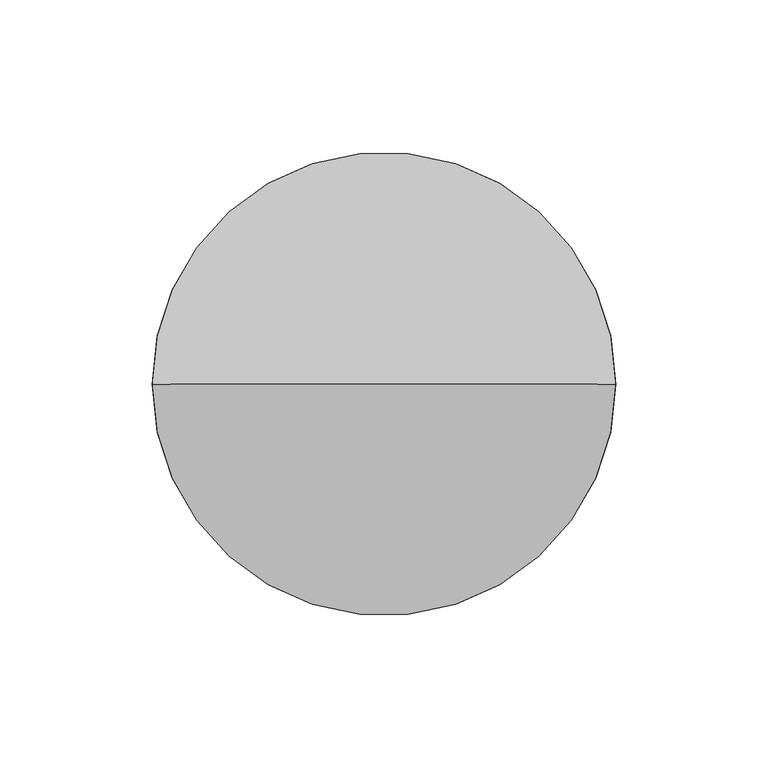
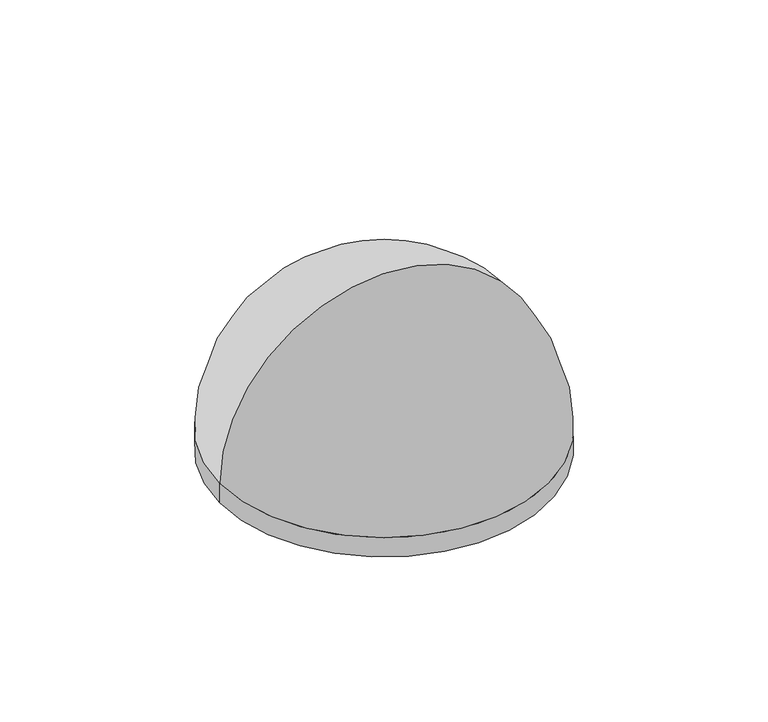
"""IFC4 building model written with IfcOpenShell, lengths in millimetres: alarm geometry, 报警闪灯 : 标准."""

from ifc_helpers import new_model, si_unit, point, frame, origin, origin_with_axes, origin_2d, place, context, project, spatial, circle_curve, ellipse_curve, trimmed, segment, composite_curve, outline, extrude, source, transform, mapped, element, save
from ifc_brep_helpers import plane_surface, revolved_surface, advanced_brep


def alarm_29ba7a31(model_context):
    return source(origin(), model_context, "Body", "SolidModel", [
        advanced_brep(
        [(0.0, 0.0, 85.5), (76.0, 0.0, 9.5), (-76.0, 0.0, 9.5), (0.0, 0.0, 9.5)],
        [
            (0, 1, circle_curve(frame((0.0, 0.0, 9.5), z_axis=(0.0, 1.0, 0.0), x_axis=(1.0, 0.0, 0.0)), 76.0)),
            (1, 2, circle_curve(frame((0.0, 0.0, 9.5), z_axis=(0.0, 0.0, 1.0), x_axis=(1.0, 0.0, 0.0)), 76.0)),
            (2, 0, circle_curve(frame((0.0, 0.0, 9.5), z_axis=(0.0, 1.0, 0.0), x_axis=(-1.0, 0.0, 0.0)), 76.0)),
            (2, 1, circle_curve(frame((0.0, 0.0, 9.5), z_axis=(0.0, 0.0, 1.0), x_axis=(1.0, 0.0, 0.0)), 76.0)),
            (1, 3),
            (3, 2),
        ],
        [
            revolved_surface(trimmed(ellipse_curve(frame((0.0, 0.0, 9.5), z_axis=(0.0, -1.0, 0.0), x_axis=(1.0, 0.0, 0.0)), 76.0, 76.0), [point((76.0, 0.0, 9.5))], [point((0.0, 0.0, 85.5))], True, "CARTESIAN"), (0.0, 0.0, 2609.0581012), (0.0, 0.0, 1.0)),
            plane_surface(frame((0.0, 0.0, 9.5), z_axis=(0.0, 0.0, -1.0), x_axis=(1.0, 0.0, 0.0))),
        ],
        [
            (0, [[1, 2, 3]]),
            (0, [[-3, 4, -1]]),
            (1, [[-2, 5, 6]]),
            (1, [[-4, -6, -5]]),
        ],
    ),
        extrude(outline(composite_curve([segment(trimmed(circle_curve(origin_2d(), 76.0), [point((-76.0, 0.0))], [point((76.0, 0.0))], False, "CARTESIAN"), True, "CONTINUOUS"), segment(trimmed(circle_curve(origin_2d(), 76.0), [point((76.0, 0.0))], [point((-76.0, 0.0))], False, "CARTESIAN"), True, "CONTINUOUS")], self_intersect=False)), origin_with_axes(), (0.0, 0.0, 1.0), 9.5),
    ])


if __name__ == "__main__":
    model = new_model("IFC4")
    model_context = context("Model", 3, world=origin())
    ifc_project = project(units=[si_unit("LENGTHUNIT", "METRE", prefix="MILLI")], contexts=[model_context])
    site = spatial("IfcSite", under=ifc_project)
    building = spatial("IfcBuilding", under=site)
    placement = place(None, origin())
    alarm_shape = alarm_29ba7a31(model_context)
    element("IfcAlarm", 1, ObjectType="报警闪灯 : 标准", at=placement, inside=building, context=model_context, shape_type="MappedRepresentation", body=[
        mapped(alarm_shape, transform((0.0, 0.0, 0.0), x_axis=(1.0, 0.0, 0.0), y_axis=(0.0, 1.0, 0.0), z_axis=(0.0, 0.0, 1.0))),
    ])
    save(model, "model.ifc")

# Revit data of these elements
# Type "报警闪灯 : 标准"
#   半径 = 76 mm
#   高度 = 9.5 mm
#   直径 = 152 mm
#   Default Elevation = 1200 mm
#   材质 = none
